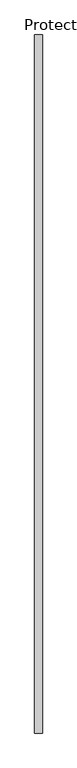
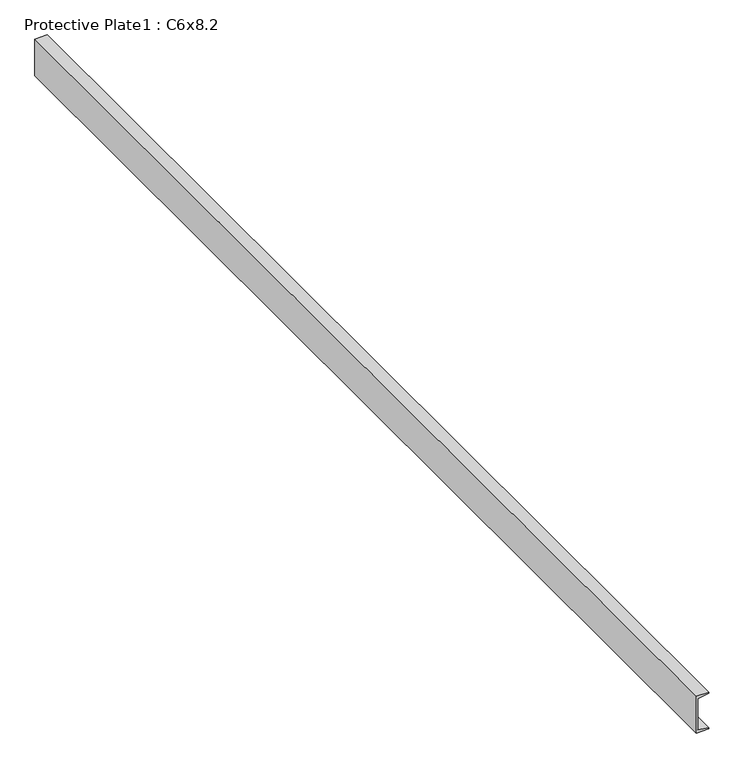
"""IFC4 building model written with IfcOpenShell, lengths in millimetres: proxy geometry, Protective Plate1 : C6x8.2."""

from ifc_helpers import new_model, si_unit, frame, origin, place, context, project, spatial, polyline, outline, extrude, source, transform, mapped, element, save


def protective_plate1_c6x8_2_0a73d697(model_context):
    return source(origin(), model_context, "Body", "SweptSolid", [
        extrude(outline(polyline([(914.4, 590217.0434739), (914.4, 590168.2754739), (762.0, 590168.2754739), (762.0, 590217.0434739), (767.08, 590217.0434739), (774.7868721, 590173.3356302), (901.6131279, 590173.3356302), (909.32, 590217.0434739), (914.4, 590217.0434739)])), frame((0.0, -536297.9573841, 0.0), z_axis=(0.0, 1.0, 0.0), x_axis=(0.0, 0.0, 1.0)), (0.0, 0.0, 1.0), 4473.448),
    ])


if __name__ == "__main__":
    model = new_model("IFC4")
    model_context = context("Model", 3, world=origin())
    ifc_project = project(units=[si_unit("LENGTHUNIT", "METRE", prefix="MILLI")], contexts=[model_context])
    site = spatial("IfcSite", under=ifc_project)
    building = spatial("IfcBuilding", under=site)
    placement = place(None, origin())
    protective_plate1_c6x8_2_shape = protective_plate1_c6x8_2_0a73d697(model_context)
    element("IfcBuildingElementProxy", 1, Name="Protective Plate1 : C6x8.2", ObjectType="Protective Plate1 : C6x8.2", at=placement, inside=building, context=model_context, shape_type="MappedRepresentation", body=[
        mapped(protective_plate1_c6x8_2_shape, transform((0.0, 0.0, 0.0), x_axis=(1.0, 0.0, 0.0), y_axis=(0.0, 1.0, 0.0), z_axis=(0.0, 0.0, 1.0))),
    ])
    save(model, "model.ifc")

# Revit data of these elements
# Element 1 (IfcBuildingElementProxy, "Protective Plate1 : C6x8.2")
#   Materials on its faces: "C6x8.2 GALV CHANNEL"
# Materials
#   "C6x8.2 GALV CHANNEL": class "Generic", colour RGB 211 211 207, transparency 0, Cost = 0
